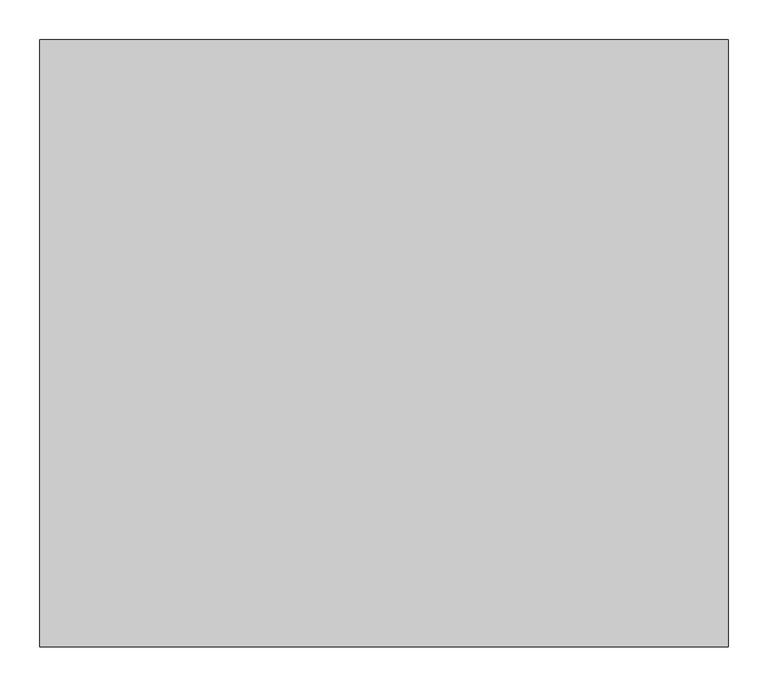
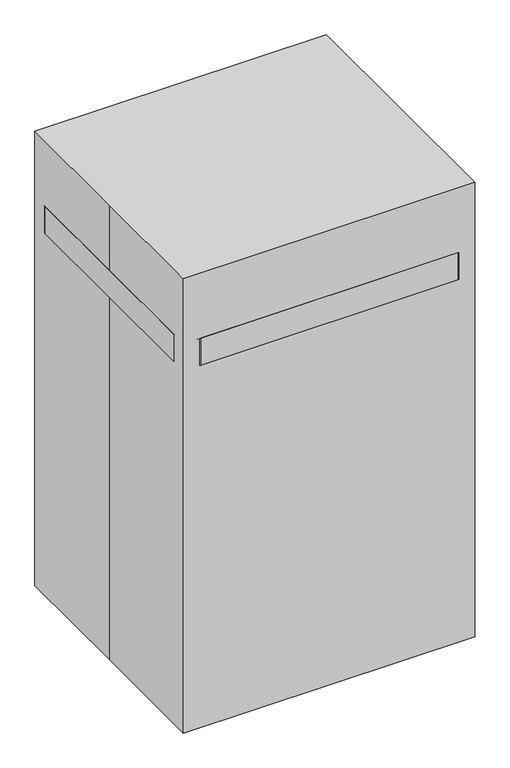
"""IFC4 building model written with IfcOpenShell, lengths in millimetres: proxy geometry, M8805 - Table, Instrument, Straddle : M8805 - Table, Instrument, Straddle."""

from ifc_helpers import new_model, si_unit, point, frame, frame_2d, origin, origin_with_axes, place, context, project, spatial, polyline, circle_curve, trimmed, segment, composite_curve, outline, extrude, source, transform, mapped, element, save


def specialty_equipment_2a4dddcc(model_context):
    return source(origin(), model_context, "Body", "SweptSolid", [
        extrude(outline(polyline([(374.65, -31.75), (311.15, -31.75), (311.15, 31.75), (374.65, 31.75), (374.65, -31.75)])), frame((0.0, 0.0, 171.69085), z_axis=(0.0, 0.0, 1.0), x_axis=(1.0, 0.0, 0.0)), (0.0, 0.0, 1.0), 277.1108167),
        extrude(outline(polyline([(381.0, -38.1), (304.8, -38.1), (304.8, 38.1), (381.0, 38.1), (381.0, -38.1)])), frame((0.0, 0.0, 448.8016667), z_axis=(0.0, 0.0, 1.0), x_axis=(1.0, 0.0, 0.0)), (0.0, 0.0, 1.0), 609.6),
        extrude(outline(polyline([(374.65, -311.15), (311.15, -311.15), (311.15, 308.1882821), (374.65, 308.1882821), (374.65, -311.15)])), frame((0.0, 0.0, 108.19085), z_axis=(0.0, 0.0, 1.0), x_axis=(1.0, 0.0, 0.0)), (0.0, 0.0, 1.0), 63.5),
        extrude(outline(polyline([(-311.15, -31.75), (-374.65, -31.75), (-374.65, 31.75), (-311.15, 31.75), (-311.15, -31.75)])), frame((0.0, 0.0, 171.69085), z_axis=(0.0, 0.0, 1.0), x_axis=(1.0, 0.0, 0.0)), (0.0, 0.0, 1.0), 277.1108167),
        extrude(outline(polyline([(-304.8, -38.1), (-381.0, -38.1), (-381.0, 38.1), (-304.8, 38.1), (-304.8, -38.1)])), frame((0.0, 0.0, 448.8016667), z_axis=(0.0, 0.0, 1.0), x_axis=(1.0, 0.0, 0.0)), (0.0, 0.0, 1.0), 609.6),
        extrude(outline(polyline([(-311.15, -311.15), (-374.65, -311.15), (-374.65, 308.1882821), (-311.15, 308.1882821), (-311.15, -311.15)])), frame((0.0, 0.0, 108.19085), z_axis=(0.0, 0.0, 1.0), x_axis=(1.0, 0.0, 0.0)), (0.0, 0.0, 1.0), 63.5),
        extrude(outline(composite_curve([segment(trimmed(circle_curve(frame_2d((50.8, -325.9666667)), 50.8), [point((50.8, -376.7666667))], [point((50.8, -275.1666667))], False, "CARTESIAN"), True, "CONTINUOUS"), segment(trimmed(circle_curve(frame_2d((50.8, -325.9666667)), 50.8), [point((50.8, -275.1666667))], [point((50.8, -376.7666667))], False, "CARTESIAN"), True, "CONTINUOUS")], self_intersect=False)), frame((0.0, -273.05, 0.0), z_axis=(0.0, 1.0, 0.0), x_axis=(0.0, 0.0, 1.0)), (0.0, 0.0, 1.0), 19.05),
        extrude(outline(composite_curve([segment(trimmed(circle_curve(frame_2d((50.8, -325.9666667)), 50.8), [point((50.8, -376.7666667))], [point((50.8, -275.1666667))], False, "CARTESIAN"), True, "CONTINUOUS"), segment(trimmed(circle_curve(frame_2d((50.8, -325.9666667)), 50.8), [point((50.8, -275.1666667))], [point((50.8, -376.7666667))], False, "CARTESIAN"), True, "CONTINUOUS")], self_intersect=False)), frame((0.0, -330.2, 0.0), z_axis=(0.0, 1.0, 0.0), x_axis=(0.0, 0.0, 1.0)), (0.0, 0.0, 1.0), 19.05),
        extrude(outline(composite_curve([segment(trimmed(circle_curve(frame_2d((-342.9, -292.1)), 16.9333333), [point((-342.9, -309.0333333))], [point((-342.9, -275.1666667))], False, "CARTESIAN"), True, "CONTINUOUS"), segment(trimmed(circle_curve(frame_2d((-342.9, -292.1)), 16.9333333), [point((-342.9, -275.1666667))], [point((-342.9, -309.0333333))], False, "CARTESIAN"), True, "CONTINUOUS")], self_intersect=False)), frame((0.0, 0.0, 50.8), z_axis=(0.0, 0.0, 1.0), x_axis=(1.0, 0.0, 0.0)), (0.0, 0.0, 1.0), 57.39085),
        extrude(outline(composite_curve([segment(trimmed(circle_curve(frame_2d((50.8, -325.9666667)), 33.8666667), [point((50.8, -292.1))], [point((50.8, -359.8333333))], False, "CARTESIAN"), True, "CONTINUOUS"), segment(trimmed(circle_curve(frame_2d((50.8, -325.9666667)), 33.8666667), [point((50.8, -359.8333333))], [point((50.8, -292.1))], False, "CARTESIAN"), True, "CONTINUOUS")], self_intersect=False)), frame((0.0, -311.15, 0.0), z_axis=(0.0, 1.0, 0.0), x_axis=(0.0, 0.0, 1.0)), (0.0, 0.0, 1.0), 38.1),
        extrude(outline(composite_curve([segment(trimmed(circle_curve(frame_2d((50.8, -325.9666667)), 50.8), [point((50.8, -376.7666667))], [point((50.8, -275.1666667))], False, "CARTESIAN"), True, "CONTINUOUS"), segment(trimmed(circle_curve(frame_2d((50.8, -325.9666667)), 50.8), [point((50.8, -275.1666667))], [point((50.8, -376.7666667))], False, "CARTESIAN"), True, "CONTINUOUS")], self_intersect=False)), frame((0.0, 251.0382821, 0.0), z_axis=(0.0, 1.0, 0.0), x_axis=(0.0, 0.0, 1.0)), (0.0, 0.0, 1.0), 19.05),
        extrude(outline(composite_curve([segment(trimmed(circle_curve(frame_2d((50.8, -325.9666667)), 50.8), [point((50.8, -376.7666667))], [point((50.8, -275.1666667))], False, "CARTESIAN"), True, "CONTINUOUS"), segment(trimmed(circle_curve(frame_2d((50.8, -325.9666667)), 50.8), [point((50.8, -275.1666667))], [point((50.8, -376.7666667))], False, "CARTESIAN"), True, "CONTINUOUS")], self_intersect=False)), frame((0.0, 308.1882821, 0.0), z_axis=(0.0, 1.0, 0.0), x_axis=(0.0, 0.0, 1.0)), (0.0, 0.0, 1.0), 19.05),
        extrude(outline(composite_curve([segment(trimmed(circle_curve(frame_2d((-342.9, 288.925)), 16.9333333), [point((-342.9, 305.8583333))], [point((-342.9, 271.9916667))], False, "CARTESIAN"), True, "CONTINUOUS"), segment(trimmed(circle_curve(frame_2d((-342.9, 288.925)), 16.9333333), [point((-342.9, 271.9916667))], [point((-342.9, 305.8583333))], False, "CARTESIAN"), True, "CONTINUOUS")], self_intersect=False)), frame((0.0, 0.0, 50.8), z_axis=(0.0, 0.0, 1.0), x_axis=(1.0, 0.0, 0.0)), (0.0, 0.0, 1.0), 57.39085),
        extrude(outline(composite_curve([segment(trimmed(circle_curve(frame_2d((50.8, -325.9666667)), 33.8666667), [point((50.8, -292.1))], [point((50.8, -359.8333333))], False, "CARTESIAN"), True, "CONTINUOUS"), segment(trimmed(circle_curve(frame_2d((50.8, -325.9666667)), 33.8666667), [point((50.8, -359.8333333))], [point((50.8, -292.1))], False, "CARTESIAN"), True, "CONTINUOUS")], self_intersect=False)), frame((0.0, 270.0882821, 0.0), z_axis=(0.0, 1.0, 0.0), x_axis=(0.0, 0.0, 1.0)), (0.0, 0.0, 1.0), 38.1),
        extrude(outline(polyline([(381.0, -254.0), (304.8, -254.0), (304.8, 251.0382821), (381.0, 251.0382821), (381.0, -254.0)])), frame((0.0, 0.0, 1058.4016667), z_axis=(0.0, 0.0, 1.0), x_axis=(1.0, 0.0, 0.0)), (0.0, 0.0, 1.0), 76.2),
        extrude(outline(polyline([(-304.8, -254.0), (-381.0, -254.0), (-381.0, 251.0382821), (-304.8, 251.0382821), (-304.8, -254.0)])), frame((0.0, 0.0, 1058.4016667), z_axis=(0.0, 0.0, 1.0), x_axis=(1.0, 0.0, 0.0)), (0.0, 0.0, 1.0), 76.2),
        extrude(outline(polyline([(381.0, -254.0), (381.0, -330.2), (-381.0, -330.2), (-381.0, -254.0), (381.0, -254.0)])), frame((0.0, 0.0, 1058.4016667), z_axis=(0.0, 0.0, 1.0), x_axis=(1.0, 0.0, 0.0)), (0.0, 0.0, 1.0), 76.2),
        extrude(outline(polyline([(381.0, 327.2382821), (381.0, 251.0382821), (-381.0, 251.0382821), (-381.0, 327.2382821), (381.0, 327.2382821)])), frame((0.0, 0.0, 1058.4016667), z_axis=(0.0, 0.0, 1.0), x_axis=(1.0, 0.0, 0.0)), (0.0, 0.0, 1.0), 76.2),
        extrude(outline(composite_curve([segment(trimmed(circle_curve(frame_2d((50.8, 325.9666667)), 50.8), [point((50.8, 376.7666667))], [point((50.8, 275.1666667))], False, "CARTESIAN"), True, "CONTINUOUS"), segment(trimmed(circle_curve(frame_2d((50.8, 325.9666667)), 50.8), [point((50.8, 275.1666667))], [point((50.8, 376.7666667))], False, "CARTESIAN"), True, "CONTINUOUS")], self_intersect=False)), frame((0.0, -273.05, 0.0), z_axis=(0.0, 1.0, 0.0), x_axis=(0.0, 0.0, 1.0)), (0.0, 0.0, 1.0), 19.05),
        extrude(outline(composite_curve([segment(trimmed(circle_curve(frame_2d((50.8, 325.9666667)), 50.8), [point((50.8, 376.7666667))], [point((50.8, 275.1666667))], False, "CARTESIAN"), True, "CONTINUOUS"), segment(trimmed(circle_curve(frame_2d((50.8, 325.9666667)), 50.8), [point((50.8, 275.1666667))], [point((50.8, 376.7666667))], False, "CARTESIAN"), True, "CONTINUOUS")], self_intersect=False)), frame((0.0, -330.2, 0.0), z_axis=(0.0, 1.0, 0.0), x_axis=(0.0, 0.0, 1.0)), (0.0, 0.0, 1.0), 19.05),
        extrude(outline(composite_curve([segment(trimmed(circle_curve(frame_2d((342.9, -292.1)), 16.9333333), [point((342.9, -309.0333333))], [point((342.9, -275.1666667))], False, "CARTESIAN"), True, "CONTINUOUS"), segment(trimmed(circle_curve(frame_2d((342.9, -292.1)), 16.9333333), [point((342.9, -275.1666667))], [point((342.9, -309.0333333))], False, "CARTESIAN"), True, "CONTINUOUS")], self_intersect=False)), frame((0.0, 0.0, 50.8), z_axis=(0.0, 0.0, 1.0), x_axis=(1.0, 0.0, 0.0)), (0.0, 0.0, 1.0), 57.39085),
        extrude(outline(composite_curve([segment(trimmed(circle_curve(frame_2d((50.8, 325.9666667)), 33.8666667), [point((50.8, 292.1))], [point((50.8, 359.8333333))], False, "CARTESIAN"), True, "CONTINUOUS"), segment(trimmed(circle_curve(frame_2d((50.8, 325.9666667)), 33.8666667), [point((50.8, 359.8333333))], [point((50.8, 292.1))], False, "CARTESIAN"), True, "CONTINUOUS")], self_intersect=False)), frame((0.0, -311.15, 0.0), z_axis=(0.0, 1.0, 0.0), x_axis=(0.0, 0.0, 1.0)), (0.0, 0.0, 1.0), 38.1),
        extrude(outline(composite_curve([segment(trimmed(circle_curve(frame_2d((50.8, 325.9666667)), 50.8), [point((50.8, 376.7666667))], [point((50.8, 275.1666667))], False, "CARTESIAN"), True, "CONTINUOUS"), segment(trimmed(circle_curve(frame_2d((50.8, 325.9666667)), 50.8), [point((50.8, 275.1666667))], [point((50.8, 376.7666667))], False, "CARTESIAN"), True, "CONTINUOUS")], self_intersect=False)), frame((0.0, 251.0382821, 0.0), z_axis=(0.0, 1.0, 0.0), x_axis=(0.0, 0.0, 1.0)), (0.0, 0.0, 1.0), 19.05),
        extrude(outline(composite_curve([segment(trimmed(circle_curve(frame_2d((50.8, 325.9666667)), 50.8), [point((50.8, 376.7666667))], [point((50.8, 275.1666667))], False, "CARTESIAN"), True, "CONTINUOUS"), segment(trimmed(circle_curve(frame_2d((50.8, 325.9666667)), 50.8), [point((50.8, 275.1666667))], [point((50.8, 376.7666667))], False, "CARTESIAN"), True, "CONTINUOUS")], self_intersect=False)), frame((0.0, 308.1882821, 0.0), z_axis=(0.0, 1.0, 0.0), x_axis=(0.0, 0.0, 1.0)), (0.0, 0.0, 1.0), 19.05),
        extrude(outline(composite_curve([segment(trimmed(circle_curve(frame_2d((342.9, 289.71875)), 16.9333333), [point((342.9, 306.6520833))], [point((342.9, 272.7854167))], False, "CARTESIAN"), True, "CONTINUOUS"), segment(trimmed(circle_curve(frame_2d((342.9, 289.71875)), 16.9333333), [point((342.9, 272.7854167))], [point((342.9, 306.6520833))], False, "CARTESIAN"), True, "CONTINUOUS")], self_intersect=False)), frame((0.0, 0.0, 50.8), z_axis=(0.0, 0.0, 1.0), x_axis=(1.0, 0.0, 0.0)), (0.0, 0.0, 1.0), 57.39085),
        extrude(outline(composite_curve([segment(trimmed(circle_curve(frame_2d((50.8, 325.9666667)), 33.8666667), [point((50.8, 292.1))], [point((50.8, 359.8333333))], False, "CARTESIAN"), True, "CONTINUOUS"), segment(trimmed(circle_curve(frame_2d((50.8, 325.9666667)), 33.8666667), [point((50.8, 359.8333333))], [point((50.8, 292.1))], False, "CARTESIAN"), True, "CONTINUOUS")], self_intersect=False)), frame((0.0, 270.0882821, 0.0), z_axis=(0.0, 1.0, 0.0), x_axis=(0.0, 0.0, 1.0)), (0.0, 0.0, 1.0), 38.1),
        extrude(outline(composite_curve([segment(trimmed(circle_curve(frame_2d((381.0, 330.2)), 50.8), [point((381.0, 381.0))], [point((431.8, 330.2))], False, "CARTESIAN"), True, "CONTINUOUS"), segment(polyline([(431.8, 330.2), (431.8, -330.2)]), True, "CONTINUOUS"), segment(trimmed(circle_curve(frame_2d((381.0, -330.2)), 50.8), [point((431.8, -330.2))], [point((381.0, -381.0))], False, "CARTESIAN"), True, "CONTINUOUS"), segment(polyline([(381.0, -381.0), (-381.0, -381.0)]), True, "CONTINUOUS"), segment(trimmed(circle_curve(frame_2d((-381.0, -330.2)), 50.8), [point((-381.0, -381.0))], [point((-431.8, -330.2))], False, "CARTESIAN"), True, "CONTINUOUS"), segment(polyline([(-431.8, -330.2), (-431.8, 330.2)]), True, "CONTINUOUS"), segment(trimmed(circle_curve(frame_2d((-381.0, 330.2)), 50.8), [point((-431.8, 330.2))], [point((-381.0, 381.0))], False, "CARTESIAN"), True, "CONTINUOUS"), segment(polyline([(-381.0, 381.0), (381.0, 381.0)]), True, "CONTINUOUS")], self_intersect=False)), frame((0.0, 0.0, 1134.6016667), z_axis=(0.0, 0.0, 1.0), x_axis=(1.0, 0.0, 0.0)), (0.0, 0.0, 1.0), 84.5983333),
        extrude(outline(polyline([(-431.8, 381.0), (431.8, 381.0), (431.8, -381.0), (-431.8, -381.0), (-431.8, 0.0), (-431.8, 381.0)])), origin_with_axes(), (0.0, 0.0, 1.0), 1422.4),
    ])


if __name__ == "__main__":
    model = new_model("IFC4")
    model_context = context("Model", 3, world=origin())
    ifc_project = project(units=[si_unit("LENGTHUNIT", "METRE", prefix="MILLI")], contexts=[model_context])
    site = spatial("IfcSite", under=ifc_project)
    building = spatial("IfcBuilding", under=site)
    placement = place(None, origin())
    specialty_equipment_shape = specialty_equipment_2a4dddcc(model_context)
    element("IfcBuildingElementProxy", 1, Name="M8805 - Table, Instrument, Straddle : M8805 - Table, Instrument, Straddle", ObjectType="M8805 - Table, Instrument, Straddle : M8805 - Table, Instrument, Straddle", at=placement, inside=building, context=model_context, shape_type="MappedRepresentation", body=[
        mapped(specialty_equipment_shape, transform((0.0, 0.0, 0.0), x_axis=(1.0, 0.0, 0.0), y_axis=(0.0, 1.0, 0.0), z_axis=(0.0, 0.0, 1.0))),
    ])
    save(model, "model.ifc")

# Revit data of these elements
# Type "M8805 - Table, Instrument, Straddle : M8805 - Table, Instrument, Straddle"
#   Watts2 = "0"
#   Watts1 = "0"
#   Unit_Issue = "EA"
#   UTIL_6_Misc = "-"
#   UTIL_5_NonMedGas = "-"
#   UTIL_4_MiscGas = "-"
#   UTIL_3_MedGas = "-"
#   UTIL_2_Elec = "-"
#   UTIL_1_WaterDrain = "-"
#   Nomenclature = "Table, Instrument, Straddle"
#   NSN = "6530"
#   Location [instance default] = ""
#   JSN = "M8805"
#   Fund_Source_VA = "-"
#   Fund_Source_Navy = "-"
#   Fund_Source_Army = "-"
#   Fund_Source_AF = "-"
#   ELEC_Volts2 = "0"
#   ELEC_Volts1 = "0"
#   ELEC_Phase2 = "0"
#   ELEC_Phase1 = "0"
#   ELEC_HertzSwitch = "0"
#   ELEC_HertzDependent = "0"
#   ELEC_Hertz = "0"
#   ELEC_Amps2 = "0"
#   ELEC_Amps1 = "0"
#   DetailDescription = "Mobile instrument/dressing table, approximately 34\" H x 20\" W x 16\" D Corrosion resistant stainless steel mobile table with sounddeadening shelf and drawer. Unit is mounted on 2\" casters. Designed for all purpose use in the hospital or clinic."
#   CAT_VA = "C"
#   CAT_Navy = "C"
#   CAT_IHS = "-"
#   CAT_Army = "C"
#   CAT_AF = "C"
#   BTUperhour = "0"
#   radius = 0' - 2"
#   calc 2 = 0' - 0.66667"
#   calc 1 = 0' - 1.33333"
#   Weight_IP = 50
#   DIM_Width_IP = 2' - 10"
#   DIM_Height_IP = 4' - 8"
#   DIM_Depth_IP = 2' - 6"
#   top [instance default] = none
#   finish [instance default] = none
# Element 1 (IfcBuildingElementProxy, "M8805 - Table, Instrument, Straddle : M8805 - Table, Instrument, Straddle")
#   Materials on its faces: "EquipSpace"
# Materials
#   "EquipSpace": class "Unassigned", colour RGB 221 217 195, transparency 0.5
